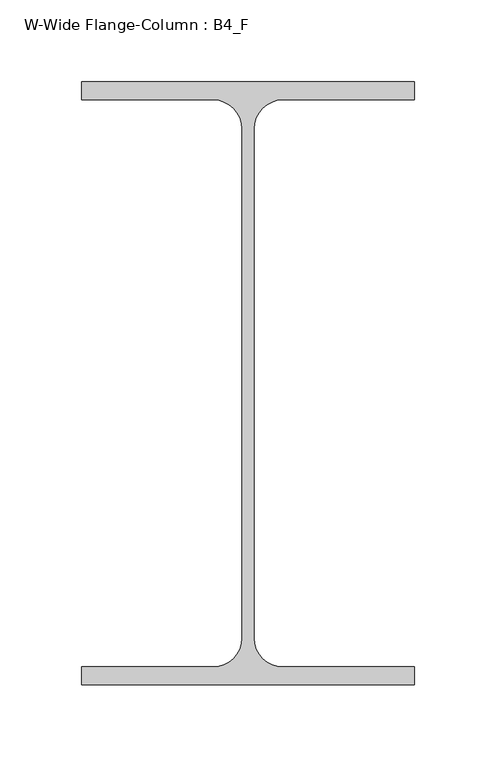
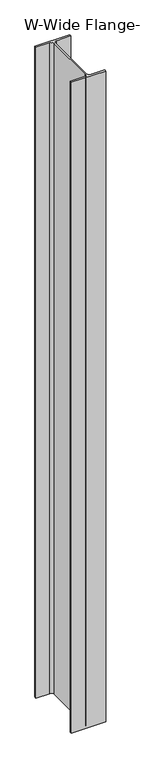
"""IFC4 building model written with IfcOpenShell, lengths in millimetres: column geometry, W-Wide Flange-Column : B4_F."""

import ifcopenshell
import ifcopenshell.guid

model = None  # the IFC model being written
_history = None  # IfcOwnerHistory: only IFC2X3 demands one
_inside = {}  # id of a spatial element -> (the spatial element, [elements in it])
_under = {}  # id of a project, library or spatial element -> (it, [spatial elements below it])
_declared = {}  # id of a project -> (the project, [libraries it declares])
_typed = {}  # id of a type object -> (the type object, [elements of that type])
_made_of = {}  # id of a material, layer set ... -> (it, [elements and type objects made of it])


def new_model(schema):
    """Start an empty IFC model of exactly this schema.

    Asked for "IFC4X3", IfcOpenShell would pick the latest addendum, in which some entities
    have other attributes; the version numbers below select the first issue.
    IFC2X3 requires an IfcOwnerHistory on every rooted entity: one is made here for all.
    """
    global model, _history
    if schema == "IFC4X3":
        model = ifcopenshell.file(schema_version=(4, 3, 0, 0))
    else:
        model = ifcopenshell.file(schema=schema)
    _inside.clear()
    _under.clear()
    _declared.clear()
    _typed.clear()
    _made_of.clear()
    _history = None
    if model.schema == "IFC2X3":
        org = make("IfcOrganization", Name="unknown")
        user = make(
            "IfcPersonAndOrganization",
            ThePerson=make("IfcPerson", FamilyName="unknown"),
            TheOrganization=org,
        )
        app = make(
            "IfcApplication",
            ApplicationDeveloper=org,
            Version="unknown",
            ApplicationFullName="unknown",
            ApplicationIdentifier="unknown",
        )
        _history = make(
            "IfcOwnerHistory",
            OwningUser=user,
            OwningApplication=app,
            ChangeAction="ADDED",
            CreationDate=0,
        )
    return model


def make(cls, **values):
    """One entity of the class cls with the attributes given. An attribute that is None is left unset."""
    return model.create_entity(
        cls, **{name: value for name, value in values.items() if value is not None}
    )


def rooted(cls, **values):
    """An entity with a GlobalId (a new one), such as an element, a storey or a relation."""
    return make(cls, GlobalId=ifcopenshell.guid.new(), OwnerHistory=_history, **values)


def si_unit(unit_type, name, prefix=None):
    """IfcSIUnit, for example si_unit("LENGTHUNIT", "METRE", prefix="MILLI")."""
    return make("IfcSIUnit", UnitType=unit_type, Prefix=prefix, Name=name)


def assignment(units):
    """IfcUnitAssignment: the units of a project."""
    return None if units is None else make("IfcUnitAssignment", Units=units)


def point(xyz):
    """IfcCartesianPoint."""
    return None if xyz is None else make("IfcCartesianPoint", Coordinates=xyz)


def direction(xyz):
    """IfcDirection."""
    return None if xyz is None else make("IfcDirection", DirectionRatios=xyz)


def frame(location, z_axis=None, x_axis=None):
    """IfcAxis2Placement3D, a coordinate frame: its origin and axes. An axis left out is left unset."""
    return make(
        "IfcAxis2Placement3D",
        Location=point(location),
        Axis=direction(z_axis),
        RefDirection=direction(x_axis),
    )


def frame_2d(location, x_axis=None):
    """IfcAxis2Placement2D, a coordinate frame in the plane: its origin and x axis."""
    return make(
        "IfcAxis2Placement2D", Location=point(location), RefDirection=direction(x_axis)
    )


def origin():
    """The frame at (0, 0, 0) with its axes left unset."""
    return frame((0.0, 0.0, 0.0))


def place(relative_to, where):
    """IfcLocalPlacement: puts the frame where relative to a parent placement (None: the world)."""
    return make(
        "IfcLocalPlacement", PlacementRelTo=relative_to, RelativePlacement=where
    )


def context(
    kind, dimensions, precision=None, world=None, true_north=None, identifier=None
):
    """IfcGeometricRepresentationContext, for example the 3D "Model" context."""
    return make(
        "IfcGeometricRepresentationContext",
        ContextIdentifier=identifier,
        ContextType=kind,
        CoordinateSpaceDimension=dimensions,
        Precision=precision,
        WorldCoordinateSystem=world,
        TrueNorth=true_north,
    )


def project(units=None, contexts=None):
    """IfcProject with its units and contexts."""
    return rooted(
        "IfcProject",
        Name="project",
        RepresentationContexts=contexts,
        UnitsInContext=assignment(units),
    )


def spatial(cls, under=None, at=None, **own):
    """A site, building, storey or space (cls), placed at a placement, below another one or the project."""
    s = rooted(cls, ObjectPlacement=at, **own)
    if under is not None:
        _under.setdefault(under.id(), (under, []))[1].append(s)
    return s


def polyline(points):
    """IfcPolyline through the points."""
    return make("IfcPolyline", Points=[point(p) for p in points])


def circle_curve(where, radius):
    """IfcCircle in the frame where."""
    return make("IfcCircle", Position=where, Radius=radius)


def trimmed(basis, trim1, trim2, sense, master):
    """IfcTrimmedCurve: the piece of a basis curve between two trims."""
    return make(
        "IfcTrimmedCurve",
        BasisCurve=basis,
        Trim1=trim1,
        Trim2=trim2,
        SenseAgreement=sense,
        MasterRepresentation=master,
    )


def segment(curve, same_sense, transition):
    """IfcCompositeCurveSegment."""
    return make(
        "IfcCompositeCurveSegment",
        Transition=transition,
        SameSense=same_sense,
        ParentCurve=curve,
    )


def composite_curve(segments, self_intersect=None):
    """IfcCompositeCurve: segments joined end to end."""
    return make("IfcCompositeCurve", Segments=segments, SelfIntersect=self_intersect)


def outline(outer, holes=None, kind="AREA"):
    """IfcArbitraryClosedProfileDef: a profile drawn as a closed curve; with holes, ...WithVoids."""
    if holes is None:
        return make("IfcArbitraryClosedProfileDef", ProfileType=kind, OuterCurve=outer)
    return make(
        "IfcArbitraryProfileDefWithVoids",
        ProfileType=kind,
        OuterCurve=outer,
        InnerCurves=holes,
    )


def extrude(swept, where, along, depth):
    """IfcExtrudedAreaSolid: the profile swept, set in the frame where, extruded along a direction by depth."""
    return make(
        "IfcExtrudedAreaSolid",
        SweptArea=swept,
        Position=where,
        ExtrudedDirection=direction(along),
        Depth=depth,
    )


def shape(context_of_items, identifier, shape_type, items):
    """IfcShapeRepresentation: the items that make up one representation, for example the "Body"."""
    return make(
        "IfcShapeRepresentation",
        ContextOfItems=context_of_items,
        RepresentationIdentifier=identifier,
        RepresentationType=shape_type,
        Items=items,
    )


def source(mapping_origin, context_of_items, identifier, shape_type, items):
    """IfcRepresentationMap: a shape defined once, which mapped items show again and again."""
    return make(
        "IfcRepresentationMap",
        MappingOrigin=mapping_origin,
        MappedRepresentation=shape(context_of_items, identifier, shape_type, items),
    )


def transform(
    local_origin,
    x_axis=None,
    y_axis=None,
    z_axis=None,
    scale=None,
    scale2=None,
    scale3=None,
    uniform=True,
):
    """IfcCartesianTransformationOperator3D, or its non-uniform kind. x_axis, y_axis, z_axis: its Axis1, 2, 3."""
    if uniform:
        return make(
            "IfcCartesianTransformationOperator3D",
            Axis1=direction(x_axis),
            Axis2=direction(y_axis),
            LocalOrigin=point(local_origin),
            Scale=scale,
            Axis3=direction(z_axis),
        )
    return make(
        "IfcCartesianTransformationOperator3DnonUniform",
        Axis1=direction(x_axis),
        Axis2=direction(y_axis),
        LocalOrigin=point(local_origin),
        Scale=scale,
        Axis3=direction(z_axis),
        Scale2=scale2,
        Scale3=scale3,
    )


def mapped(mapping_source, mapping_target):
    """IfcMappedItem: shows the shape of a source again, moved by a transform."""
    return make(
        "IfcMappedItem", MappingSource=mapping_source, MappingTarget=mapping_target
    )


def made_of(thing, what):
    """Note that an element or type object is made of a material, layer set ...; save() writes the relation."""
    if what is not None:
        _made_of.setdefault(what.id(), (what, []))[1].append(thing)
    return thing


def element(
    cls,
    number,
    at=None,
    inside=None,
    cuts=None,
    type_object=None,
    material=None,
    context=None,
    identifier="Body",
    shape_type=None,
    held_by="IfcProductDefinitionShape",
    body=None,
    shapes=None,
    **own,
):
    """One element of the class cls, such as IfcWall. Its Tag is "e" and its number.

    at: its placement. inside: the storey or other place that contains it. cuts: it is an
    opening in that element (IfcRelVoidsElement). A single representation is given by context,
    identifier, shape_type and body (its items); several are given by shapes. held_by: the class
    of the entity that holds the representations. save() writes the other relations.
    """
    e = rooted(cls, Tag="e%d" % number, ObjectPlacement=at, **own)
    if body is not None:
        shapes = [shape(context, identifier, shape_type, body)]
    if shapes is not None:
        e.Representation = make(held_by, Representations=shapes)
    if inside is not None:
        _inside.setdefault(inside.id(), (inside, []))[1].append(e)
    if cuts is not None:
        rooted(
            "IfcRelVoidsElement", RelatingBuildingElement=cuts, RelatedOpeningElement=e
        )
    if type_object is not None:
        _typed.setdefault(type_object.id(), (type_object, []))[1].append(e)
    return made_of(e, material)


def aggregate(whole, parts):
    """IfcRelAggregates: a whole, such as a stair, and the parts it consists of."""
    return rooted("IfcRelAggregates", RelatingObject=whole, RelatedObjects=parts)


def save(model, path):
    """Write the relations noted so far, then the file.

    IfcRelAggregates (storeys below a building ...), IfcRelContainedInSpatialStructure (elements
    in a storey), IfcRelDefinesByType, IfcRelAssociatesMaterial and IfcRelDeclares: one each for
    every whole, place, type object, material and project.
    """
    for whole, parts in _under.values():
        aggregate(whole, parts)
    for where, things in _inside.values():
        rooted(
            "IfcRelContainedInSpatialStructure",
            RelatedElements=things,
            RelatingStructure=where,
        )
    for kind, things in _typed.values():
        rooted("IfcRelDefinesByType", RelatedObjects=things, RelatingType=kind)
    for what, things in _made_of.values():
        rooted("IfcRelAssociatesMaterial", RelatedObjects=things, RelatingMaterial=what)
    for by, libraries in _declared.values():
        rooted("IfcRelDeclares", RelatingContext=by, RelatedDefinitions=libraries)
    model.write(path)


def w_wide_flange_column_b4_f_8a8a01a4(model_context):
    return source(origin(), model_context, "Body", "SweptSolid", [
        extrude(outline(composite_curve([segment(polyline([(101.6, 184.15), (101.6, 173.1367188), (21.2328125, 173.1367188)]), True, "CONTINUOUS"), segment(trimmed(circle_curve(frame_2d((21.2328125, 155.575)), 17.5617188), [point((21.2328125, 173.1367188))], [point((3.6710937, 155.575))], True, "CARTESIAN"), True, "CONTINUOUS"), segment(polyline([(3.6710937, 155.575), (3.6710937, -155.575)]), True, "CONTINUOUS"), segment(trimmed(circle_curve(frame_2d((21.2328125, -155.575)), 17.5617188), [point((3.6710937, -155.575))], [point((21.2328125, -173.1367187))], True, "CARTESIAN"), True, "CONTINUOUS"), segment(polyline([(21.2328125, -173.1367187), (101.6, -173.1367187), (101.6, -184.15), (-101.6, -184.15), (-101.6, -173.1367187), (-21.2328125, -173.1367187)]), True, "CONTINUOUS"), segment(trimmed(circle_curve(frame_2d((-21.2328125, -155.575)), 17.5617188), [point((-21.2328125, -173.1367187))], [point((-3.6710938, -155.575))], True, "CARTESIAN"), True, "CONTINUOUS"), segment(polyline([(-3.6710938, -155.575), (-3.6710938, 155.575)]), True, "CONTINUOUS"), segment(trimmed(circle_curve(frame_2d((-21.2328125, 155.575)), 17.5617188), [point((-3.6710938, 155.575))], [point((-21.2328125, 173.1367188))], True, "CARTESIAN"), True, "CONTINUOUS"), segment(polyline([(-21.2328125, 173.1367188), (-101.6, 173.1367188), (-101.6, 184.15), (101.6, 184.15)]), True, "CONTINUOUS")], self_intersect=False)), frame((0.0, 0.0, -304.8), z_axis=(0.0, 0.0, 1.0), x_axis=(1.0, 0.0, 0.0)), (0.0, 0.0, 1.0), 4025.9),
    ])


if __name__ == "__main__":
    model = new_model("IFC4")
    model_context = context("Model", 3, world=origin())
    ifc_project = project(units=[si_unit("LENGTHUNIT", "METRE", prefix="MILLI")], contexts=[model_context])
    site = spatial("IfcSite", under=ifc_project)
    building = spatial("IfcBuilding", under=site)
    placement = place(None, origin())
    w_wide_flange_column_b4_f_shape = w_wide_flange_column_b4_f_8a8a01a4(model_context)
    element("IfcColumn", 1, ObjectType="W-Wide Flange-Column : B4_F", at=placement, inside=building, context=model_context, shape_type="MappedRepresentation", body=[
        mapped(w_wide_flange_column_b4_f_shape, transform((0.0, 0.0, 0.0), x_axis=(1.0, 0.0, 0.0), y_axis=(0.0, 1.0, 0.0), z_axis=(0.0, 0.0, 1.0))),
    ])
    save(model, "model.ifc")

# Revit data of these elements
# Type "W-Wide Flange-Column : B4_F"
#   Assembly Code = "B10"
#   W = 33
#   bf = 0' - 8"
#   d = 1' - 2 1/2"
#   k = 0' - 1 1/8"
#   kr = 0' - 0 177/256"
#   tf = 0' - 0 111/256"
#   tw = 0' - 0 37/128"
#   A = 0.07 SF
#   Structural Material [instance default] = Steel ASTM A992
# Element 1 (IfcColumn, "W-Wide Flange-Column : B4_F")
#   Structural Material = STRUCTURAL STEEL - SEE STRUCT. DWGS
#   Materials on its faces: "STRUCTURAL STEEL - SEE STRUCT. DWGS"
# Materials
#   "Steel ASTM A992": class "Metal", colour RGB 199 199 199, transparency 0, Description = "Structural steel 50ksi", Cost = 0
#   "STRUCTURAL STEEL - SEE STRUCT. DWGS": class "Metal", colour RGB 137 146 153, transparency 0, Description = "Steel, mill finish", Cost = 0
